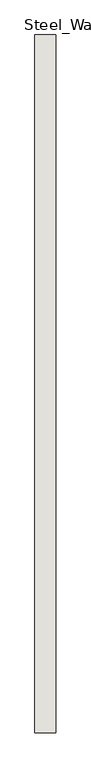
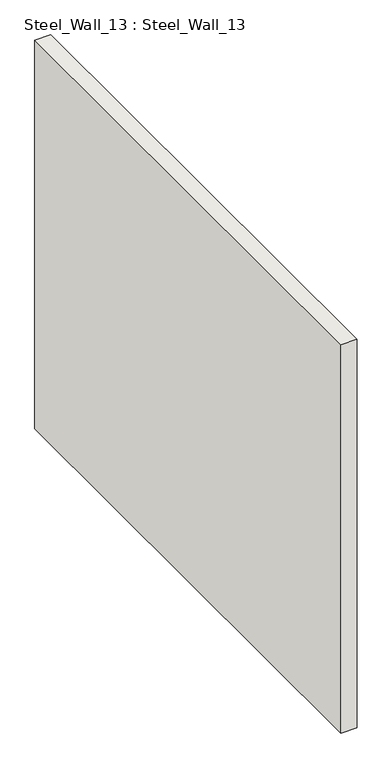
"""IFC4 building model written with IfcOpenShell, lengths in millimetres: wall geometry, Steel_Wall_13 : Steel_Wall_13."""

import ifcopenshell
import ifcopenshell.guid

model = None  # the IFC model being written
_history = None  # IfcOwnerHistory: only IFC2X3 demands one
_inside = {}  # id of a spatial element -> (the spatial element, [elements in it])
_under = {}  # id of a project, library or spatial element -> (it, [spatial elements below it])
_declared = {}  # id of a project -> (the project, [libraries it declares])
_typed = {}  # id of a type object -> (the type object, [elements of that type])
_made_of = {}  # id of a material, layer set ... -> (it, [elements and type objects made of it])


def new_model(schema):
    """Start an empty IFC model of exactly this schema.

    Asked for "IFC4X3", IfcOpenShell would pick the latest addendum, in which some entities
    have other attributes; the version numbers below select the first issue.
    IFC2X3 requires an IfcOwnerHistory on every rooted entity: one is made here for all.
    """
    global model, _history
    if schema == "IFC4X3":
        model = ifcopenshell.file(schema_version=(4, 3, 0, 0))
    else:
        model = ifcopenshell.file(schema=schema)
    _inside.clear()
    _under.clear()
    _declared.clear()
    _typed.clear()
    _made_of.clear()
    _history = None
    if model.schema == "IFC2X3":
        org = make("IfcOrganization", Name="unknown")
        user = make(
            "IfcPersonAndOrganization",
            ThePerson=make("IfcPerson", FamilyName="unknown"),
            TheOrganization=org,
        )
        app = make(
            "IfcApplication",
            ApplicationDeveloper=org,
            Version="unknown",
            ApplicationFullName="unknown",
            ApplicationIdentifier="unknown",
        )
        _history = make(
            "IfcOwnerHistory",
            OwningUser=user,
            OwningApplication=app,
            ChangeAction="ADDED",
            CreationDate=0,
        )
    return model


def make(cls, **values):
    """One entity of the class cls with the attributes given. An attribute that is None is left unset."""
    return model.create_entity(
        cls, **{name: value for name, value in values.items() if value is not None}
    )


def rooted(cls, **values):
    """An entity with a GlobalId (a new one), such as an element, a storey or a relation."""
    return make(cls, GlobalId=ifcopenshell.guid.new(), OwnerHistory=_history, **values)


def si_unit(unit_type, name, prefix=None):
    """IfcSIUnit, for example si_unit("LENGTHUNIT", "METRE", prefix="MILLI")."""
    return make("IfcSIUnit", UnitType=unit_type, Prefix=prefix, Name=name)


def assignment(units):
    """IfcUnitAssignment: the units of a project."""
    return None if units is None else make("IfcUnitAssignment", Units=units)


def point(xyz):
    """IfcCartesianPoint."""
    return None if xyz is None else make("IfcCartesianPoint", Coordinates=xyz)


def direction(xyz):
    """IfcDirection."""
    return None if xyz is None else make("IfcDirection", DirectionRatios=xyz)


def frame(location, z_axis=None, x_axis=None):
    """IfcAxis2Placement3D, a coordinate frame: its origin and axes. An axis left out is left unset."""
    return make(
        "IfcAxis2Placement3D",
        Location=point(location),
        Axis=direction(z_axis),
        RefDirection=direction(x_axis),
    )


def origin():
    """The frame at (0, 0, 0) with its axes left unset."""
    return frame((0.0, 0.0, 0.0))


def place(relative_to, where):
    """IfcLocalPlacement: puts the frame where relative to a parent placement (None: the world)."""
    return make(
        "IfcLocalPlacement", PlacementRelTo=relative_to, RelativePlacement=where
    )


def context(
    kind, dimensions, precision=None, world=None, true_north=None, identifier=None
):
    """IfcGeometricRepresentationContext, for example the 3D "Model" context."""
    return make(
        "IfcGeometricRepresentationContext",
        ContextIdentifier=identifier,
        ContextType=kind,
        CoordinateSpaceDimension=dimensions,
        Precision=precision,
        WorldCoordinateSystem=world,
        TrueNorth=true_north,
    )


def project(units=None, contexts=None):
    """IfcProject with its units and contexts."""
    return rooted(
        "IfcProject",
        Name="project",
        RepresentationContexts=contexts,
        UnitsInContext=assignment(units),
    )


def spatial(cls, under=None, at=None, **own):
    """A site, building, storey or space (cls), placed at a placement, below another one or the project."""
    s = rooted(cls, ObjectPlacement=at, **own)
    if under is not None:
        _under.setdefault(under.id(), (under, []))[1].append(s)
    return s


def polyline(points):
    """IfcPolyline through the points."""
    return make("IfcPolyline", Points=[point(p) for p in points])


def outline(outer, holes=None, kind="AREA"):
    """IfcArbitraryClosedProfileDef: a profile drawn as a closed curve; with holes, ...WithVoids."""
    if holes is None:
        return make("IfcArbitraryClosedProfileDef", ProfileType=kind, OuterCurve=outer)
    return make(
        "IfcArbitraryProfileDefWithVoids",
        ProfileType=kind,
        OuterCurve=outer,
        InnerCurves=holes,
    )


def extrude(swept, where, along, depth):
    """IfcExtrudedAreaSolid: the profile swept, set in the frame where, extruded along a direction by depth."""
    return make(
        "IfcExtrudedAreaSolid",
        SweptArea=swept,
        Position=where,
        ExtrudedDirection=direction(along),
        Depth=depth,
    )


def shape(context_of_items, identifier, shape_type, items):
    """IfcShapeRepresentation: the items that make up one representation, for example the "Body"."""
    return make(
        "IfcShapeRepresentation",
        ContextOfItems=context_of_items,
        RepresentationIdentifier=identifier,
        RepresentationType=shape_type,
        Items=items,
    )


def source(mapping_origin, context_of_items, identifier, shape_type, items):
    """IfcRepresentationMap: a shape defined once, which mapped items show again and again."""
    return make(
        "IfcRepresentationMap",
        MappingOrigin=mapping_origin,
        MappedRepresentation=shape(context_of_items, identifier, shape_type, items),
    )


def transform(
    local_origin,
    x_axis=None,
    y_axis=None,
    z_axis=None,
    scale=None,
    scale2=None,
    scale3=None,
    uniform=True,
):
    """IfcCartesianTransformationOperator3D, or its non-uniform kind. x_axis, y_axis, z_axis: its Axis1, 2, 3."""
    if uniform:
        return make(
            "IfcCartesianTransformationOperator3D",
            Axis1=direction(x_axis),
            Axis2=direction(y_axis),
            LocalOrigin=point(local_origin),
            Scale=scale,
            Axis3=direction(z_axis),
        )
    return make(
        "IfcCartesianTransformationOperator3DnonUniform",
        Axis1=direction(x_axis),
        Axis2=direction(y_axis),
        LocalOrigin=point(local_origin),
        Scale=scale,
        Axis3=direction(z_axis),
        Scale2=scale2,
        Scale3=scale3,
    )


def mapped(mapping_source, mapping_target):
    """IfcMappedItem: shows the shape of a source again, moved by a transform."""
    return make(
        "IfcMappedItem", MappingSource=mapping_source, MappingTarget=mapping_target
    )


def made_of(thing, what):
    """Note that an element or type object is made of a material, layer set ...; save() writes the relation."""
    if what is not None:
        _made_of.setdefault(what.id(), (what, []))[1].append(thing)
    return thing


def element(
    cls,
    number,
    at=None,
    inside=None,
    cuts=None,
    type_object=None,
    material=None,
    context=None,
    identifier="Body",
    shape_type=None,
    held_by="IfcProductDefinitionShape",
    body=None,
    shapes=None,
    **own,
):
    """One element of the class cls, such as IfcWall. Its Tag is "e" and its number.

    at: its placement. inside: the storey or other place that contains it. cuts: it is an
    opening in that element (IfcRelVoidsElement). A single representation is given by context,
    identifier, shape_type and body (its items); several are given by shapes. held_by: the class
    of the entity that holds the representations. save() writes the other relations.
    """
    e = rooted(cls, Tag="e%d" % number, ObjectPlacement=at, **own)
    if body is not None:
        shapes = [shape(context, identifier, shape_type, body)]
    if shapes is not None:
        e.Representation = make(held_by, Representations=shapes)
    if inside is not None:
        _inside.setdefault(inside.id(), (inside, []))[1].append(e)
    if cuts is not None:
        rooted(
            "IfcRelVoidsElement", RelatingBuildingElement=cuts, RelatedOpeningElement=e
        )
    if type_object is not None:
        _typed.setdefault(type_object.id(), (type_object, []))[1].append(e)
    return made_of(e, material)


def aggregate(whole, parts):
    """IfcRelAggregates: a whole, such as a stair, and the parts it consists of."""
    return rooted("IfcRelAggregates", RelatingObject=whole, RelatedObjects=parts)


def save(model, path):
    """Write the relations noted so far, then the file.

    IfcRelAggregates (storeys below a building ...), IfcRelContainedInSpatialStructure (elements
    in a storey), IfcRelDefinesByType, IfcRelAssociatesMaterial and IfcRelDeclares: one each for
    every whole, place, type object, material and project.
    """
    for whole, parts in _under.values():
        aggregate(whole, parts)
    for where, things in _inside.values():
        rooted(
            "IfcRelContainedInSpatialStructure",
            RelatedElements=things,
            RelatingStructure=where,
        )
    for kind, things in _typed.values():
        rooted("IfcRelDefinesByType", RelatedObjects=things, RelatingType=kind)
    for what, things in _made_of.values():
        rooted("IfcRelAssociatesMaterial", RelatedObjects=things, RelatingMaterial=what)
    for by, libraries in _declared.values():
        rooted("IfcRelDeclares", RelatingContext=by, RelatedDefinitions=libraries)
    model.write(path)


def steel_wall_13_steel_wall_13_94e184f7(model_context):
    return source(origin(), model_context, "Body", "SweptSolid", [
        extrude(outline(polyline([(4925.0, 3755.0), (4925.0, 395.0), (4825.0, 395.0), (4825.0, 3755.0), (4925.0, 3755.0)])), frame((0.0, 0.0, 250.0), z_axis=(0.0, 0.0, 1.0), x_axis=(1.0, 0.0, 0.0)), (0.0, 0.0, 1.0), 2600.0),
    ])


if __name__ == "__main__":
    model = new_model("IFC4")
    model_context = context("Model", 3, world=origin())
    ifc_project = project(units=[si_unit("LENGTHUNIT", "METRE", prefix="MILLI")], contexts=[model_context])
    site = spatial("IfcSite", under=ifc_project)
    building = spatial("IfcBuilding", under=site)
    placement = place(None, origin())
    steel_wall_13_steel_wall_13_shape = steel_wall_13_steel_wall_13_94e184f7(model_context)
    element("IfcWall", 1, ObjectType="Steel_Wall_13 : Steel_Wall_13", at=placement, inside=building, context=model_context, shape_type="MappedRepresentation", body=[
        mapped(steel_wall_13_steel_wall_13_shape, transform((0.0, 0.0, 0.0), x_axis=(1.0, 0.0, 0.0), y_axis=(0.0, 1.0, 0.0), z_axis=(0.0, 0.0, 1.0))),
    ])
    save(model, "model.ifc")

# Revit data of these elements
# Type "Steel_Wall_13 : Steel_Wall_13"
#   NameOverride = "Steel_Wall_13"
# Element 1 (IfcWall, "Steel_Wall_13 : Steel_Wall_13")
#   Materials on its faces: "IfcSurfaceStyle #33"
# Materials
#   "IfcSurfaceStyle #33": class "Unassigned", colour RGB 214 214 214, transparency 0
